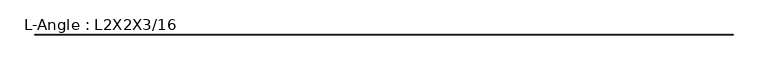
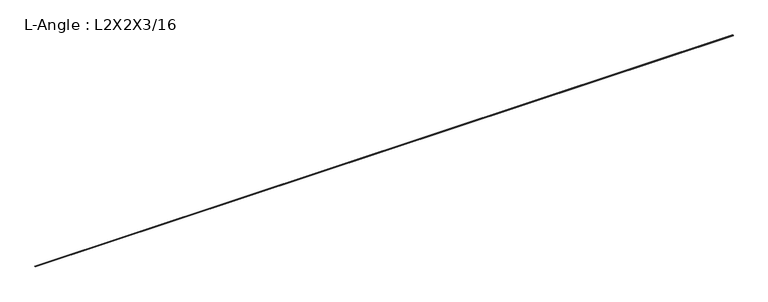
"""IFC4 building model written with IfcOpenShell, lengths in millimetres: beam geometry, L-Angle : L2X2X3/16."""

import ifcopenshell
import ifcopenshell.guid

model = None  # the IFC model being written
_history = None  # IfcOwnerHistory: only IFC2X3 demands one
_inside = {}  # id of a spatial element -> (the spatial element, [elements in it])
_under = {}  # id of a project, library or spatial element -> (it, [spatial elements below it])
_declared = {}  # id of a project -> (the project, [libraries it declares])
_typed = {}  # id of a type object -> (the type object, [elements of that type])
_made_of = {}  # id of a material, layer set ... -> (it, [elements and type objects made of it])


def new_model(schema):
    """Start an empty IFC model of exactly this schema.

    Asked for "IFC4X3", IfcOpenShell would pick the latest addendum, in which some entities
    have other attributes; the version numbers below select the first issue.
    IFC2X3 requires an IfcOwnerHistory on every rooted entity: one is made here for all.
    """
    global model, _history
    if schema == "IFC4X3":
        model = ifcopenshell.file(schema_version=(4, 3, 0, 0))
    else:
        model = ifcopenshell.file(schema=schema)
    _inside.clear()
    _under.clear()
    _declared.clear()
    _typed.clear()
    _made_of.clear()
    _history = None
    if model.schema == "IFC2X3":
        org = make("IfcOrganization", Name="unknown")
        user = make(
            "IfcPersonAndOrganization",
            ThePerson=make("IfcPerson", FamilyName="unknown"),
            TheOrganization=org,
        )
        app = make(
            "IfcApplication",
            ApplicationDeveloper=org,
            Version="unknown",
            ApplicationFullName="unknown",
            ApplicationIdentifier="unknown",
        )
        _history = make(
            "IfcOwnerHistory",
            OwningUser=user,
            OwningApplication=app,
            ChangeAction="ADDED",
            CreationDate=0,
        )
    return model


def make(cls, **values):
    """One entity of the class cls with the attributes given. An attribute that is None is left unset."""
    return model.create_entity(
        cls, **{name: value for name, value in values.items() if value is not None}
    )


def rooted(cls, **values):
    """An entity with a GlobalId (a new one), such as an element, a storey or a relation."""
    return make(cls, GlobalId=ifcopenshell.guid.new(), OwnerHistory=_history, **values)


def si_unit(unit_type, name, prefix=None):
    """IfcSIUnit, for example si_unit("LENGTHUNIT", "METRE", prefix="MILLI")."""
    return make("IfcSIUnit", UnitType=unit_type, Prefix=prefix, Name=name)


def assignment(units):
    """IfcUnitAssignment: the units of a project."""
    return None if units is None else make("IfcUnitAssignment", Units=units)


def point(xyz):
    """IfcCartesianPoint."""
    return None if xyz is None else make("IfcCartesianPoint", Coordinates=xyz)


def direction(xyz):
    """IfcDirection."""
    return None if xyz is None else make("IfcDirection", DirectionRatios=xyz)


def frame(location, z_axis=None, x_axis=None):
    """IfcAxis2Placement3D, a coordinate frame: its origin and axes. An axis left out is left unset."""
    return make(
        "IfcAxis2Placement3D",
        Location=point(location),
        Axis=direction(z_axis),
        RefDirection=direction(x_axis),
    )


def frame_2d(location, x_axis=None):
    """IfcAxis2Placement2D, a coordinate frame in the plane: its origin and x axis."""
    return make(
        "IfcAxis2Placement2D", Location=point(location), RefDirection=direction(x_axis)
    )


def origin():
    """The frame at (0, 0, 0) with its axes left unset."""
    return frame((0.0, 0.0, 0.0))


def place(relative_to, where):
    """IfcLocalPlacement: puts the frame where relative to a parent placement (None: the world)."""
    return make(
        "IfcLocalPlacement", PlacementRelTo=relative_to, RelativePlacement=where
    )


def context(
    kind, dimensions, precision=None, world=None, true_north=None, identifier=None
):
    """IfcGeometricRepresentationContext, for example the 3D "Model" context."""
    return make(
        "IfcGeometricRepresentationContext",
        ContextIdentifier=identifier,
        ContextType=kind,
        CoordinateSpaceDimension=dimensions,
        Precision=precision,
        WorldCoordinateSystem=world,
        TrueNorth=true_north,
    )


def project(units=None, contexts=None):
    """IfcProject with its units and contexts."""
    return rooted(
        "IfcProject",
        Name="project",
        RepresentationContexts=contexts,
        UnitsInContext=assignment(units),
    )


def spatial(cls, under=None, at=None, **own):
    """A site, building, storey or space (cls), placed at a placement, below another one or the project."""
    s = rooted(cls, ObjectPlacement=at, **own)
    if under is not None:
        _under.setdefault(under.id(), (under, []))[1].append(s)
    return s


def polyline(points):
    """IfcPolyline through the points."""
    return make("IfcPolyline", Points=[point(p) for p in points])


def circle_curve(where, radius):
    """IfcCircle in the frame where."""
    return make("IfcCircle", Position=where, Radius=radius)


def trimmed(basis, trim1, trim2, sense, master):
    """IfcTrimmedCurve: the piece of a basis curve between two trims."""
    return make(
        "IfcTrimmedCurve",
        BasisCurve=basis,
        Trim1=trim1,
        Trim2=trim2,
        SenseAgreement=sense,
        MasterRepresentation=master,
    )


def segment(curve, same_sense, transition):
    """IfcCompositeCurveSegment."""
    return make(
        "IfcCompositeCurveSegment",
        Transition=transition,
        SameSense=same_sense,
        ParentCurve=curve,
    )


def composite_curve(segments, self_intersect=None):
    """IfcCompositeCurve: segments joined end to end."""
    return make("IfcCompositeCurve", Segments=segments, SelfIntersect=self_intersect)


def outline(outer, holes=None, kind="AREA"):
    """IfcArbitraryClosedProfileDef: a profile drawn as a closed curve; with holes, ...WithVoids."""
    if holes is None:
        return make("IfcArbitraryClosedProfileDef", ProfileType=kind, OuterCurve=outer)
    return make(
        "IfcArbitraryProfileDefWithVoids",
        ProfileType=kind,
        OuterCurve=outer,
        InnerCurves=holes,
    )


def extrude(swept, where, along, depth):
    """IfcExtrudedAreaSolid: the profile swept, set in the frame where, extruded along a direction by depth."""
    return make(
        "IfcExtrudedAreaSolid",
        SweptArea=swept,
        Position=where,
        ExtrudedDirection=direction(along),
        Depth=depth,
    )


def shape(context_of_items, identifier, shape_type, items):
    """IfcShapeRepresentation: the items that make up one representation, for example the "Body"."""
    return make(
        "IfcShapeRepresentation",
        ContextOfItems=context_of_items,
        RepresentationIdentifier=identifier,
        RepresentationType=shape_type,
        Items=items,
    )


def source(mapping_origin, context_of_items, identifier, shape_type, items):
    """IfcRepresentationMap: a shape defined once, which mapped items show again and again."""
    return make(
        "IfcRepresentationMap",
        MappingOrigin=mapping_origin,
        MappedRepresentation=shape(context_of_items, identifier, shape_type, items),
    )


def transform(
    local_origin,
    x_axis=None,
    y_axis=None,
    z_axis=None,
    scale=None,
    scale2=None,
    scale3=None,
    uniform=True,
):
    """IfcCartesianTransformationOperator3D, or its non-uniform kind. x_axis, y_axis, z_axis: its Axis1, 2, 3."""
    if uniform:
        return make(
            "IfcCartesianTransformationOperator3D",
            Axis1=direction(x_axis),
            Axis2=direction(y_axis),
            LocalOrigin=point(local_origin),
            Scale=scale,
            Axis3=direction(z_axis),
        )
    return make(
        "IfcCartesianTransformationOperator3DnonUniform",
        Axis1=direction(x_axis),
        Axis2=direction(y_axis),
        LocalOrigin=point(local_origin),
        Scale=scale,
        Axis3=direction(z_axis),
        Scale2=scale2,
        Scale3=scale3,
    )


def mapped(mapping_source, mapping_target):
    """IfcMappedItem: shows the shape of a source again, moved by a transform."""
    return make(
        "IfcMappedItem", MappingSource=mapping_source, MappingTarget=mapping_target
    )


def made_of(thing, what):
    """Note that an element or type object is made of a material, layer set ...; save() writes the relation."""
    if what is not None:
        _made_of.setdefault(what.id(), (what, []))[1].append(thing)
    return thing


def element(
    cls,
    number,
    at=None,
    inside=None,
    cuts=None,
    type_object=None,
    material=None,
    context=None,
    identifier="Body",
    shape_type=None,
    held_by="IfcProductDefinitionShape",
    body=None,
    shapes=None,
    **own,
):
    """One element of the class cls, such as IfcWall. Its Tag is "e" and its number.

    at: its placement. inside: the storey or other place that contains it. cuts: it is an
    opening in that element (IfcRelVoidsElement). A single representation is given by context,
    identifier, shape_type and body (its items); several are given by shapes. held_by: the class
    of the entity that holds the representations. save() writes the other relations.
    """
    e = rooted(cls, Tag="e%d" % number, ObjectPlacement=at, **own)
    if body is not None:
        shapes = [shape(context, identifier, shape_type, body)]
    if shapes is not None:
        e.Representation = make(held_by, Representations=shapes)
    if inside is not None:
        _inside.setdefault(inside.id(), (inside, []))[1].append(e)
    if cuts is not None:
        rooted(
            "IfcRelVoidsElement", RelatingBuildingElement=cuts, RelatedOpeningElement=e
        )
    if type_object is not None:
        _typed.setdefault(type_object.id(), (type_object, []))[1].append(e)
    return made_of(e, material)


def aggregate(whole, parts):
    """IfcRelAggregates: a whole, such as a stair, and the parts it consists of."""
    return rooted("IfcRelAggregates", RelatingObject=whole, RelatedObjects=parts)


def save(model, path):
    """Write the relations noted so far, then the file.

    IfcRelAggregates (storeys below a building ...), IfcRelContainedInSpatialStructure (elements
    in a storey), IfcRelDefinesByType, IfcRelAssociatesMaterial and IfcRelDeclares: one each for
    every whole, place, type object, material and project.
    """
    for whole, parts in _under.values():
        aggregate(whole, parts)
    for where, things in _inside.values():
        rooted(
            "IfcRelContainedInSpatialStructure",
            RelatedElements=things,
            RelatingStructure=where,
        )
    for kind, things in _typed.values():
        rooted("IfcRelDefinesByType", RelatedObjects=things, RelatingType=kind)
    for what, things in _made_of.values():
        rooted("IfcRelAssociatesMaterial", RelatedObjects=things, RelatingMaterial=what)
    for by, libraries in _declared.values():
        rooted("IfcRelDeclares", RelatingContext=by, RelatedDefinitions=libraries)
    model.write(path)


def l_angle_l2x2x3_16_9da130ac(model_context):
    return source(origin(), model_context, "Body", "SweptSolid", [
        extrude(outline(composite_curve([segment(polyline([(-14.2494, 14.2494), (36.5506, 14.2494)]), True, "CONTINUOUS"), segment(trimmed(circle_curve(frame_2d((31.7881, 14.2494)), 4.7625), [point((36.5506, 14.2494))], [point((31.7881, 9.4869))], False, "CARTESIAN"), True, "CONTINUOUS"), segment(polyline([(31.7881, 9.4869), (-4.7244, 9.4869)]), True, "CONTINUOUS"), segment(trimmed(circle_curve(frame_2d((-4.7244, 4.7244)), 4.7625), [point((-4.7244, 9.4869))], [point((-9.4869, 4.7244))], True, "CARTESIAN"), True, "CONTINUOUS"), segment(polyline([(-9.4869, 4.7244), (-9.4869, -31.7881)]), True, "CONTINUOUS"), segment(trimmed(circle_curve(frame_2d((-14.2494, -31.7881)), 4.7625), [point((-9.4869, -31.7881))], [point((-14.2494, -36.5506))], False, "CARTESIAN"), True, "CONTINUOUS"), segment(polyline([(-14.2494, -36.5506), (-14.2494, 14.2494)]), True, "CONTINUOUS")], self_intersect=False)), frame((-44322.7519531, 0.0, 0.0), z_axis=(1.0, 0.0, 0.0), x_axis=(0.0, 1.0, 0.0)), (0.0, 0.0, 1.0), 88645.5039063),
    ])


if __name__ == "__main__":
    model = new_model("IFC4")
    model_context = context("Model", 3, world=origin())
    ifc_project = project(units=[si_unit("LENGTHUNIT", "METRE", prefix="MILLI")], contexts=[model_context])
    site = spatial("IfcSite", under=ifc_project)
    building = spatial("IfcBuilding", under=site)
    placement = place(None, origin())
    l_angle_l2x2x3_16_shape = l_angle_l2x2x3_16_9da130ac(model_context)
    element("IfcBeam", 1, ObjectType="L-Angle : L2X2X3/16", at=placement, inside=building, context=model_context, shape_type="MappedRepresentation", body=[
        mapped(l_angle_l2x2x3_16_shape, transform((0.0, 0.0, 0.0), x_axis=(1.0, 0.0, 0.0), y_axis=(0.0, 1.0, 0.0), z_axis=(0.0, 0.0, 1.0))),
    ])
    save(model, "model.ifc")

# Revit data of these elements
# Type "L-Angle : L2X2X3/16"
#   Assembly Code = "B10"
#   k = 0' - 0 7/16"
#   W = 2.44
#   Start Extension Calculation [instance default] = 10' - 0"
#   Start Extension [instance default] = -0' - 0 1/2"
#   End Extension Calculation [instance default] = 10' - 0"
#   End Extension [instance default] = -0' - 0 1/2"
#   Length [instance default] = 5' - 0"
#   b = 0' - 2"
#   d = 0' - 2"
#   t = 0' - 0 3/16"
#   x = 0' - 0.561"
#   y = 0' - 0.561"
#   A = 0.00496528 SF
#   Structural Material [instance default] = Metal - Steel - ASTM A36
# Element 1 (IfcBeam, "L-Angle : L2X2X3/16")
#   Structural Material = STRUCTURAL STEEL - SEE STRUCT. DWGS
#   Materials on its faces: "STRUCTURAL STEEL - SEE STRUCT. DWGS"
# Materials
#   "Metal - Steel - ASTM A36": class "Metal", colour RGB 199 199 199, transparency 0
#   "STRUCTURAL STEEL - SEE STRUCT. DWGS": class "Metal", colour RGB 137 146 153, transparency 0, Description = "Steel, mill finish", Cost = 0
